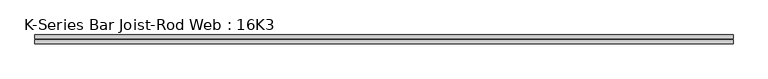
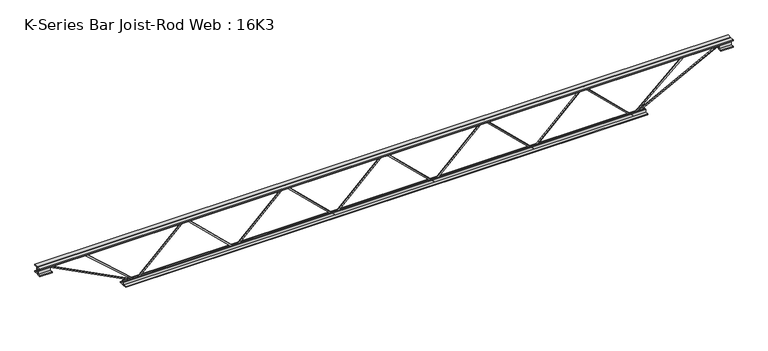
"""IFC4 building model written with IfcOpenShell, lengths in millimetres: beam geometry, K-Series Bar Joist-Rod Web : 16K3."""

from ifc_helpers import new_model, si_unit, frame, origin, place, context, project, spatial, polyline, outline, extrude, source, transform, mapped, element, save


def k_series_bar_joist_rod_web_16k3_07e5b19b(model_context):
    return source(origin(), model_context, "Body", "SweptSolid", [
        extrude(outline(polyline([(-192.0875, 413.54375), (-201.6125, 413.54375), (-201.6125, 418.6446051), (192.0875, 825.8383551), (192.0875, 828.3366449), (-201.6125, 1235.5303949), (-201.6125, 1240.63125), (-192.0875, 1240.63125), (-192.0875, 1239.3821051), (201.6125, 832.1883551), (201.6125, 821.9866449), (-192.0875, 414.7928949), (-192.0875, 413.54375)])), frame((0.0, -4.7625, 0.0), z_axis=(0.0, 1.0, 0.0), x_axis=(0.0, 0.0, 1.0)), (0.0, 0.0, 1.0), 9.525),
        extrude(outline(polyline([(-192.0875, -413.54375), (-201.6125, -413.54375), (-201.6125, -408.4428949), (192.0875, -1.2491449), (192.0875, 1.2491449), (-201.6125, 408.4428949), (-201.6125, 413.54375), (-192.0875, 413.54375), (-192.0875, 412.2946051), (201.6125, 5.1008551), (201.6125, -5.1008551), (-192.0875, -412.2946051), (-192.0875, -413.54375)])), frame((0.0, -4.7625, 0.0), z_axis=(0.0, 1.0, 0.0), x_axis=(0.0, 0.0, 1.0)), (0.0, 0.0, 1.0), 9.525),
        extrude(outline(polyline([(-192.0875, -1240.63125), (-201.6125, -1240.63125), (-201.6125, -1235.5303949), (192.0875, -828.3366449), (192.0875, -825.8383551), (-201.6125, -418.6446051), (-201.6125, -413.54375), (-192.0875, -413.54375), (-192.0875, -414.7928949), (201.6125, -821.9866449), (201.6125, -832.1883551), (-192.0875, -1239.3821051), (-192.0875, -1240.63125)])), frame((0.0, -4.7625, 0.0), z_axis=(0.0, 1.0, 0.0), x_axis=(0.0, 0.0, 1.0)), (0.0, 0.0, 1.0), 9.525),
        extrude(outline(polyline([(-192.0875, 1240.63125), (-201.6125, 1240.63125), (-201.6125, 1245.7321051), (192.0875, 1652.9258551), (192.0875, 1655.4241449), (-201.6125, 2062.6178949), (-201.6125, 2067.71875), (-192.0875, 2067.71875), (-192.0875, 2066.4696051), (201.6125, 1659.2758551), (201.6125, 1649.0741449), (-192.0875, 1241.8803949), (-192.0875, 1240.63125)])), frame((0.0, -4.7625, 0.0), z_axis=(0.0, 1.0, 0.0), x_axis=(0.0, 0.0, 1.0)), (0.0, 0.0, 1.0), 9.525),
        extrude(outline(polyline([(-192.0875, -2067.71875), (-201.6125, -2067.71875), (-201.6125, -2062.6178949), (192.0875, -1655.4241449), (192.0875, -1652.9258551), (-201.6125, -1245.7321051), (-201.6125, -1240.63125), (-192.0875, -1240.63125), (-192.0875, -1241.8803949), (201.6125, -1649.0741449), (201.6125, -1659.2758551), (-192.0875, -2066.4696051), (-192.0875, -2067.71875)])), frame((0.0, -4.7625, 0.0), z_axis=(0.0, 1.0, 0.0), x_axis=(0.0, 0.0, 1.0)), (0.0, 0.0, 1.0), 9.525),
        extrude(outline(polyline([(4.7625, 203.2), (36.5125, 203.2), (36.5125, 196.85), (11.1125, 196.85), (11.1125, 171.45), (4.7625, 171.45), (4.7625, 203.2)])), frame((-2880.51875, 0.0, 0.0), z_axis=(1.0, 0.0, 0.0), x_axis=(0.0, 1.0, 0.0)), (0.0, 0.0, 1.0), 5761.0375),
        extrude(outline(polyline([(-4.7625, 203.2), (-4.7625, 171.45), (-11.1125, 171.45), (-11.1125, 196.85), (-36.5125, 196.85), (-36.5125, 203.2), (-4.7625, 203.2)])), frame((-2880.51875, 0.0, 0.0), z_axis=(1.0, 0.0, 0.0), x_axis=(0.0, 1.0, 0.0)), (0.0, 0.0, 1.0), 5761.0375),
        extrude(outline(polyline([(-4.7625, 139.7), (-36.5125, 139.7), (-36.5125, 146.05), (-11.1125, 146.05), (-11.1125, 171.45), (-4.7625, 171.45), (-4.7625, 139.7)])), frame((-2880.51875, 0.0, 0.0), z_axis=(1.0, 0.0, 0.0), x_axis=(0.0, 1.0, 0.0)), (0.0, 0.0, 1.0), 101.6),
        extrude(outline(polyline([(36.5125, 139.7), (4.7625, 139.7), (4.7625, 171.45), (11.1125, 171.45), (11.1125, 146.05), (36.5125, 146.05), (36.5125, 139.7)])), frame((-2880.51875, 0.0, 0.0), z_axis=(1.0, 0.0, 0.0), x_axis=(0.0, 1.0, 0.0)), (0.0, 0.0, 1.0), 101.6),
        extrude(outline(polyline([(4.7625, 139.7), (4.7625, 171.45), (11.1125, 171.45), (11.1125, 146.05), (36.5125, 146.05), (36.5125, 139.7), (4.7625, 139.7)])), frame((2778.91875, 0.0, 0.0), z_axis=(1.0, 0.0, 0.0), x_axis=(0.0, 1.0, 0.0)), (0.0, 0.0, 1.0), 101.6),
        extrude(outline(polyline([(-4.7625, 139.7), (-36.5125, 139.7), (-36.5125, 146.05), (-11.1125, 146.05), (-11.1125, 171.45), (-4.7625, 171.45), (-4.7625, 139.7)])), frame((2778.91875, 0.0, 0.0), z_axis=(1.0, 0.0, 0.0), x_axis=(0.0, 1.0, 0.0)), (0.0, 0.0, 1.0), 101.6),
        extrude(outline(polyline([(4.7625, -203.2), (4.7625, -171.45), (11.1125, -171.45), (11.1125, -196.85), (36.5125, -196.85), (36.5125, -203.2), (4.7625, -203.2)])), frame((-2169.31875, 0.0, 0.0), z_axis=(1.0, 0.0, 0.0), x_axis=(0.0, 1.0, 0.0)), (0.0, 0.0, 1.0), 4338.6375),
        extrude(outline(polyline([(-4.7625, -203.2), (-36.5125, -203.2), (-36.5125, -196.85), (-11.1125, -196.85), (-11.1125, -171.45), (-4.7625, -171.45), (-4.7625, -203.2)])), frame((-2169.31875, 0.0, 0.0), z_axis=(1.0, 0.0, 0.0), x_axis=(0.0, 1.0, 0.0)), (0.0, 0.0, 1.0), 4338.6375),
        extrude(outline(polyline([(0.0, -9.525), (0.0, 0.0), (800.9059433, 0.0), (800.9059433, -9.525), (0.0, -9.525)])), frame((-2781.1088059, 4.7625, 167.2209266), z_axis=(0.45985424766113703, 0.0, 0.8879944092774513), x_axis=(0.8879944092774513, 0.0, -0.45985424766113703)), (0.0, 0.0, 1.0), 9.525),
        extrude(outline(polyline([(0.0, -9.525), (0.0, 0.0), (553.7719054, 0.0), (553.7719054, -9.525), (0.0, -9.525)])), frame((-2484.429921, 4.7625, 167.8934777), z_axis=(0.6650752709485992, 0.0, 0.7467763279407345), x_axis=(0.7467763279407345, 0.0, -0.6650752709485992)), (0.0, 0.0, 1.0), 9.525),
        extrude(outline(polyline([(0.0, -9.525), (0.0, 0.0), (800.9059433, 0.0), (800.9059433, -9.525), (0.0, -9.525)])), frame((2781.1088059, -4.7625, 167.2209266), z_axis=(-0.4598542476611245, 0.0, 0.8879944092774579), x_axis=(-0.8879944092774579, 0.0, -0.4598542476611245)), (0.0, 0.0, 1.0), 9.525),
        extrude(outline(polyline([(0.0, -9.525), (0.0, 0.0), (553.7719054, 0.0), (553.7719054, -9.525), (0.0, -9.525)])), frame((2484.429921, -4.7625, 167.8934777), z_axis=(-0.665075270948596, 0.0, 0.7467763279407374), x_axis=(-0.7467763279407374, 0.0, -0.665075270948596)), (0.0, 0.0, 1.0), 9.525),
    ])


if __name__ == "__main__":
    model = new_model("IFC4")
    model_context = context("Model", 3, world=origin())
    ifc_project = project(units=[si_unit("LENGTHUNIT", "METRE", prefix="MILLI")], contexts=[model_context])
    site = spatial("IfcSite", under=ifc_project)
    building = spatial("IfcBuilding", under=site)
    placement = place(None, origin())
    k_series_bar_joist_rod_web_16k3_shape = k_series_bar_joist_rod_web_16k3_07e5b19b(model_context)
    element("IfcBeam", 1, ObjectType="K-Series Bar Joist-Rod Web : 16K3", at=placement, inside=building, context=model_context, shape_type="MappedRepresentation", body=[
        mapped(k_series_bar_joist_rod_web_16k3_shape, transform((0.0, 0.0, 0.0), x_axis=(1.0, 0.0, 0.0), y_axis=(0.0, 1.0, 0.0), z_axis=(0.0, 0.0, 1.0))),
    ])
    save(model, "model.ifc")

# Revit data of these elements
# Type "K-Series Bar Joist-Rod Web : 16K3"
#   Assembly Code = "B1010350"
#   Wt = 6.3
#   Web Thickness = 0' - 0 3/8"
#   Start Offset [instance default] = 0' - 0"
#   Start Extension [instance default] = 0' - 0"
#   Seat Length = 0' - 4"
#   Seat Depth = 0' - 2 1/2"
#   PanelArrayLength [instance default] = 18' - 8"
#   Panel [instance default] = 2' - 8"
#   End Offset [instance default] = 0' - 0"
#   End Extension [instance default] = 0' - 0"
#   End Panel = 2' - 8"
#   Cord Leg = 0' - 1 1/4"
#   Chord Thickness = 0' - 0 1/4"
#   Length [instance default] = 24' - 0"
#   Depth = 1' - 4"
#   PanelArrayNum [instance default] = 7
#   Structural Material = none
# Element 1 (IfcBeam, "K-Series Bar Joist-Rod Web : 16K3")
#   PanelArrayLength = 13' - 6 13/16"
#   Panel = 2' - 8 9/16"
#   PanelArrayNum = 5
